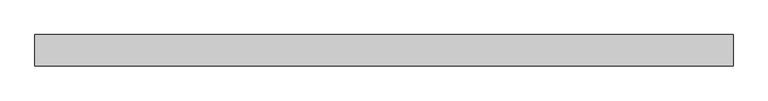
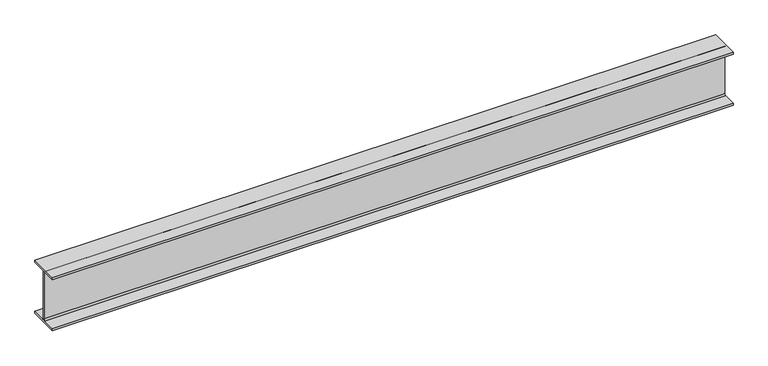
"""IFC4 building model written with IfcOpenShell, lengths in millimetres: beam geometry, Old_Steel Beam_H-KSD3502 : H_SB_ASB_H-200×200x8x12."""

import ifcopenshell
import ifcopenshell.guid

model = None  # the IFC model being written
_history = None  # IfcOwnerHistory: only IFC2X3 demands one
_inside = {}  # id of a spatial element -> (the spatial element, [elements in it])
_under = {}  # id of a project, library or spatial element -> (it, [spatial elements below it])
_declared = {}  # id of a project -> (the project, [libraries it declares])
_typed = {}  # id of a type object -> (the type object, [elements of that type])
_made_of = {}  # id of a material, layer set ... -> (it, [elements and type objects made of it])


def new_model(schema):
    """Start an empty IFC model of exactly this schema.

    Asked for "IFC4X3", IfcOpenShell would pick the latest addendum, in which some entities
    have other attributes; the version numbers below select the first issue.
    IFC2X3 requires an IfcOwnerHistory on every rooted entity: one is made here for all.
    """
    global model, _history
    if schema == "IFC4X3":
        model = ifcopenshell.file(schema_version=(4, 3, 0, 0))
    else:
        model = ifcopenshell.file(schema=schema)
    _inside.clear()
    _under.clear()
    _declared.clear()
    _typed.clear()
    _made_of.clear()
    _history = None
    if model.schema == "IFC2X3":
        org = make("IfcOrganization", Name="unknown")
        user = make(
            "IfcPersonAndOrganization",
            ThePerson=make("IfcPerson", FamilyName="unknown"),
            TheOrganization=org,
        )
        app = make(
            "IfcApplication",
            ApplicationDeveloper=org,
            Version="unknown",
            ApplicationFullName="unknown",
            ApplicationIdentifier="unknown",
        )
        _history = make(
            "IfcOwnerHistory",
            OwningUser=user,
            OwningApplication=app,
            ChangeAction="ADDED",
            CreationDate=0,
        )
    return model


def make(cls, **values):
    """One entity of the class cls with the attributes given. An attribute that is None is left unset."""
    return model.create_entity(
        cls, **{name: value for name, value in values.items() if value is not None}
    )


def rooted(cls, **values):
    """An entity with a GlobalId (a new one), such as an element, a storey or a relation."""
    return make(cls, GlobalId=ifcopenshell.guid.new(), OwnerHistory=_history, **values)


def si_unit(unit_type, name, prefix=None):
    """IfcSIUnit, for example si_unit("LENGTHUNIT", "METRE", prefix="MILLI")."""
    return make("IfcSIUnit", UnitType=unit_type, Prefix=prefix, Name=name)


def assignment(units):
    """IfcUnitAssignment: the units of a project."""
    return None if units is None else make("IfcUnitAssignment", Units=units)


def point(xyz):
    """IfcCartesianPoint."""
    return None if xyz is None else make("IfcCartesianPoint", Coordinates=xyz)


def direction(xyz):
    """IfcDirection."""
    return None if xyz is None else make("IfcDirection", DirectionRatios=xyz)


def frame(location, z_axis=None, x_axis=None):
    """IfcAxis2Placement3D, a coordinate frame: its origin and axes. An axis left out is left unset."""
    return make(
        "IfcAxis2Placement3D",
        Location=point(location),
        Axis=direction(z_axis),
        RefDirection=direction(x_axis),
    )


def frame_2d(location, x_axis=None):
    """IfcAxis2Placement2D, a coordinate frame in the plane: its origin and x axis."""
    return make(
        "IfcAxis2Placement2D", Location=point(location), RefDirection=direction(x_axis)
    )


def origin():
    """The frame at (0, 0, 0) with its axes left unset."""
    return frame((0.0, 0.0, 0.0))


def place(relative_to, where):
    """IfcLocalPlacement: puts the frame where relative to a parent placement (None: the world)."""
    return make(
        "IfcLocalPlacement", PlacementRelTo=relative_to, RelativePlacement=where
    )


def context(
    kind, dimensions, precision=None, world=None, true_north=None, identifier=None
):
    """IfcGeometricRepresentationContext, for example the 3D "Model" context."""
    return make(
        "IfcGeometricRepresentationContext",
        ContextIdentifier=identifier,
        ContextType=kind,
        CoordinateSpaceDimension=dimensions,
        Precision=precision,
        WorldCoordinateSystem=world,
        TrueNorth=true_north,
    )


def project(units=None, contexts=None):
    """IfcProject with its units and contexts."""
    return rooted(
        "IfcProject",
        Name="project",
        RepresentationContexts=contexts,
        UnitsInContext=assignment(units),
    )


def spatial(cls, under=None, at=None, **own):
    """A site, building, storey or space (cls), placed at a placement, below another one or the project."""
    s = rooted(cls, ObjectPlacement=at, **own)
    if under is not None:
        _under.setdefault(under.id(), (under, []))[1].append(s)
    return s


def polyline(points):
    """IfcPolyline through the points."""
    return make("IfcPolyline", Points=[point(p) for p in points])


def circle_curve(where, radius):
    """IfcCircle in the frame where."""
    return make("IfcCircle", Position=where, Radius=radius)


def trimmed(basis, trim1, trim2, sense, master):
    """IfcTrimmedCurve: the piece of a basis curve between two trims."""
    return make(
        "IfcTrimmedCurve",
        BasisCurve=basis,
        Trim1=trim1,
        Trim2=trim2,
        SenseAgreement=sense,
        MasterRepresentation=master,
    )


def segment(curve, same_sense, transition):
    """IfcCompositeCurveSegment."""
    return make(
        "IfcCompositeCurveSegment",
        Transition=transition,
        SameSense=same_sense,
        ParentCurve=curve,
    )


def composite_curve(segments, self_intersect=None):
    """IfcCompositeCurve: segments joined end to end."""
    return make("IfcCompositeCurve", Segments=segments, SelfIntersect=self_intersect)


def outline(outer, holes=None, kind="AREA"):
    """IfcArbitraryClosedProfileDef: a profile drawn as a closed curve; with holes, ...WithVoids."""
    if holes is None:
        return make("IfcArbitraryClosedProfileDef", ProfileType=kind, OuterCurve=outer)
    return make(
        "IfcArbitraryProfileDefWithVoids",
        ProfileType=kind,
        OuterCurve=outer,
        InnerCurves=holes,
    )


def extrude(swept, where, along, depth):
    """IfcExtrudedAreaSolid: the profile swept, set in the frame where, extruded along a direction by depth."""
    return make(
        "IfcExtrudedAreaSolid",
        SweptArea=swept,
        Position=where,
        ExtrudedDirection=direction(along),
        Depth=depth,
    )


def shape(context_of_items, identifier, shape_type, items):
    """IfcShapeRepresentation: the items that make up one representation, for example the "Body"."""
    return make(
        "IfcShapeRepresentation",
        ContextOfItems=context_of_items,
        RepresentationIdentifier=identifier,
        RepresentationType=shape_type,
        Items=items,
    )


def source(mapping_origin, context_of_items, identifier, shape_type, items):
    """IfcRepresentationMap: a shape defined once, which mapped items show again and again."""
    return make(
        "IfcRepresentationMap",
        MappingOrigin=mapping_origin,
        MappedRepresentation=shape(context_of_items, identifier, shape_type, items),
    )


def transform(
    local_origin,
    x_axis=None,
    y_axis=None,
    z_axis=None,
    scale=None,
    scale2=None,
    scale3=None,
    uniform=True,
):
    """IfcCartesianTransformationOperator3D, or its non-uniform kind. x_axis, y_axis, z_axis: its Axis1, 2, 3."""
    if uniform:
        return make(
            "IfcCartesianTransformationOperator3D",
            Axis1=direction(x_axis),
            Axis2=direction(y_axis),
            LocalOrigin=point(local_origin),
            Scale=scale,
            Axis3=direction(z_axis),
        )
    return make(
        "IfcCartesianTransformationOperator3DnonUniform",
        Axis1=direction(x_axis),
        Axis2=direction(y_axis),
        LocalOrigin=point(local_origin),
        Scale=scale,
        Axis3=direction(z_axis),
        Scale2=scale2,
        Scale3=scale3,
    )


def mapped(mapping_source, mapping_target):
    """IfcMappedItem: shows the shape of a source again, moved by a transform."""
    return make(
        "IfcMappedItem", MappingSource=mapping_source, MappingTarget=mapping_target
    )


def made_of(thing, what):
    """Note that an element or type object is made of a material, layer set ...; save() writes the relation."""
    if what is not None:
        _made_of.setdefault(what.id(), (what, []))[1].append(thing)
    return thing


def element(
    cls,
    number,
    at=None,
    inside=None,
    cuts=None,
    type_object=None,
    material=None,
    context=None,
    identifier="Body",
    shape_type=None,
    held_by="IfcProductDefinitionShape",
    body=None,
    shapes=None,
    **own,
):
    """One element of the class cls, such as IfcWall. Its Tag is "e" and its number.

    at: its placement. inside: the storey or other place that contains it. cuts: it is an
    opening in that element (IfcRelVoidsElement). A single representation is given by context,
    identifier, shape_type and body (its items); several are given by shapes. held_by: the class
    of the entity that holds the representations. save() writes the other relations.
    """
    e = rooted(cls, Tag="e%d" % number, ObjectPlacement=at, **own)
    if body is not None:
        shapes = [shape(context, identifier, shape_type, body)]
    if shapes is not None:
        e.Representation = make(held_by, Representations=shapes)
    if inside is not None:
        _inside.setdefault(inside.id(), (inside, []))[1].append(e)
    if cuts is not None:
        rooted(
            "IfcRelVoidsElement", RelatingBuildingElement=cuts, RelatedOpeningElement=e
        )
    if type_object is not None:
        _typed.setdefault(type_object.id(), (type_object, []))[1].append(e)
    return made_of(e, material)


def aggregate(whole, parts):
    """IfcRelAggregates: a whole, such as a stair, and the parts it consists of."""
    return rooted("IfcRelAggregates", RelatingObject=whole, RelatedObjects=parts)


def save(model, path):
    """Write the relations noted so far, then the file.

    IfcRelAggregates (storeys below a building ...), IfcRelContainedInSpatialStructure (elements
    in a storey), IfcRelDefinesByType, IfcRelAssociatesMaterial and IfcRelDeclares: one each for
    every whole, place, type object, material and project.
    """
    for whole, parts in _under.values():
        aggregate(whole, parts)
    for where, things in _inside.values():
        rooted(
            "IfcRelContainedInSpatialStructure",
            RelatedElements=things,
            RelatingStructure=where,
        )
    for kind, things in _typed.values():
        rooted("IfcRelDefinesByType", RelatedObjects=things, RelatingType=kind)
    for what, things in _made_of.values():
        rooted("IfcRelAssociatesMaterial", RelatedObjects=things, RelatingMaterial=what)
    for by, libraries in _declared.values():
        rooted("IfcRelDeclares", RelatingContext=by, RelatedDefinitions=libraries)
    model.write(path)


def beam_9a490488(model_context):
    return source(origin(), model_context, "Body", "SweptSolid", [
        extrude(outline(composite_curve([segment(polyline([(-82.5, -141.5), (-11.9, -141.5)]), True, "CONTINUOUS"), segment(trimmed(circle_curve(frame_2d((-11.9, -132.6)), 8.9), [point((-11.9, -141.5))], [point((-3.0, -132.6))], True, "CARTESIAN"), True, "CONTINUOUS"), segment(polyline([(-3.0, -132.6), (-3.0, 132.6)]), True, "CONTINUOUS"), segment(trimmed(circle_curve(frame_2d((-11.9, 132.6)), 8.9), [point((-3.0, 132.6))], [point((-11.9, 141.5))], True, "CARTESIAN"), True, "CONTINUOUS"), segment(polyline([(-11.9, 141.5), (-82.5, 141.5), (-82.5, 151.7), (82.5, 151.7), (82.5, 141.5), (11.9, 141.5)]), True, "CONTINUOUS"), segment(trimmed(circle_curve(frame_2d((11.9, 132.6)), 8.9), [point((11.9, 141.5))], [point((3.0, 132.6))], True, "CARTESIAN"), True, "CONTINUOUS"), segment(polyline([(3.0, 132.6), (3.0, -132.6)]), True, "CONTINUOUS"), segment(trimmed(circle_curve(frame_2d((11.9, -132.6)), 8.9), [point((3.0, -132.6))], [point((11.9, -141.5))], True, "CARTESIAN"), True, "CONTINUOUS"), segment(polyline([(11.9, -141.5), (82.5, -141.5), (82.5, -151.7), (-82.5, -151.7), (-82.5, -141.5)]), True, "CONTINUOUS")], self_intersect=False)), frame((-1872.8032895, 0.0, 0.0), z_axis=(1.0, 0.0, 0.0), x_axis=(0.0, 1.0, 0.0)), (0.0, 0.0, 1.0), 3693.2731785),
    ])


if __name__ == "__main__":
    model = new_model("IFC4")
    model_context = context("Model", 3, world=origin())
    ifc_project = project(units=[si_unit("LENGTHUNIT", "METRE", prefix="MILLI")], contexts=[model_context])
    site = spatial("IfcSite", under=ifc_project)
    building = spatial("IfcBuilding", under=site)
    placement = place(None, origin())
    beam_shape = beam_9a490488(model_context)
    element("IfcBeam", 1, ObjectType="Old_Steel Beam_H-KSD3502 : H_SB_ASB_H-200×200x8x12", at=placement, inside=building, context=model_context, shape_type="MappedRepresentation", body=[
        mapped(beam_shape, transform((0.0, 0.0, 0.0), x_axis=(1.0, 0.0, 0.0), y_axis=(0.0, 1.0, 0.0), z_axis=(0.0, 0.0, 1.0))),
    ])
    save(model, "model.ifc")

# Revit data of these elements
# Type "Old_Steel Beam_H-KSD3502 : H_SB_ASB_H-200×200x8x12"
#   Width = 20.0 cm
#   Web Thickness = 0.8 cm
#   Web Fillet = 1.3 cm
#   Warping Constant = 141376.0 cm⁶
#   Torsional Moment of Inertia = 26.2485 cm⁴
#   Torsional Modulus = 1.0 cm³
#   Section Area = 63.53 cm²
#   Plastic Modulus weak axis = 244.0 cm³
#   Plastic Modulus strong axis = 525.0 cm³
#   Perimeter = 1.16 m²/m
#   Nominal Weight = 49.90 kgf/m
#   Moment of Inertia weak axis = 1600.00 cm⁴
#   Moment of Inertia strong axis = 4720.00 cm⁴
#   Height = 20.0 cm
#   Flange Thickness = 1.2 cm
#   Elastic Modulus weak axis = 160.0 cm³
#   Elastic Modulus strong axis = 472.0 cm³
#   Centroid Vertical = 10.0 cm
#   Centroid Horizontal = 10.0 cm
#   Length [instance default] = 1.5240 m
#   Structural Material [instance default] = Steel, 45-345
#   Assembly Code = ""
# Element 1 (IfcBeam, "Old_Steel Beam_H-KSD3502 : H_SB_ASB_H-200×200x8x12")
#   Structural Material = none
# Materials
#   "Steel, 45-345": class "Metal", colour RGB 189 187 185, transparency 0, Description = "Steel 345 MPa", Cost = 0
